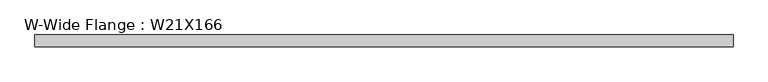
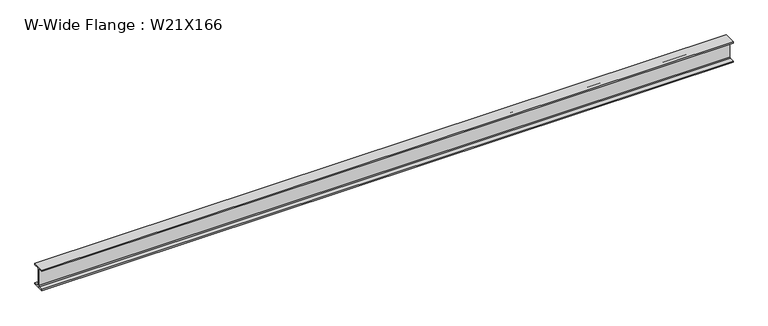
"""IFC4 building model written with IfcOpenShell, lengths in millimetres: beam geometry, W-Wide Flange : W21X166."""

from ifc_helpers import new_model, si_unit, point, frame, frame_2d, origin, place, context, project, spatial, polyline, circle_curve, trimmed, segment, composite_curve, outline, extrude, source, transform, mapped, element, save


def w_wide_flange_w21x166_b0166a6a(model_context):
    return source(origin(), model_context, "Body", "SweptSolid", [
        extrude(outline(composite_curve([segment(polyline([(157.48, -251.206), (157.48, -285.75), (-157.48, -285.75), (-157.48, -251.206), (-32.131, -251.206)]), True, "CONTINUOUS"), segment(trimmed(circle_curve(frame_2d((-32.131, -228.6)), 22.606), [point((-32.131, -251.206))], [point((-9.525, -228.6))], True, "CARTESIAN"), True, "CONTINUOUS"), segment(polyline([(-9.525, -228.6), (-9.525, 228.6)]), True, "CONTINUOUS"), segment(trimmed(circle_curve(frame_2d((-32.131, 228.6)), 22.606), [point((-9.525, 228.6))], [point((-32.131, 251.206))], True, "CARTESIAN"), True, "CONTINUOUS"), segment(polyline([(-32.131, 251.206), (-157.48, 251.206), (-157.48, 285.75), (157.48, 285.75), (157.48, 251.206), (32.131, 251.206)]), True, "CONTINUOUS"), segment(trimmed(circle_curve(frame_2d((32.131, 228.6)), 22.606), [point((32.131, 251.206))], [point((9.525, 228.6))], True, "CARTESIAN"), True, "CONTINUOUS"), segment(polyline([(9.525, 228.6), (9.525, -228.6)]), True, "CONTINUOUS"), segment(trimmed(circle_curve(frame_2d((32.131, -228.6)), 22.606), [point((9.525, -228.6))], [point((32.131, -251.206))], True, "CARTESIAN"), True, "CONTINUOUS"), segment(polyline([(32.131, -251.206), (157.48, -251.206)]), True, "CONTINUOUS")], self_intersect=False)), frame((-9106.3295465, 0.0, 0.0), z_axis=(1.0, 0.0, 0.0), x_axis=(0.0, 1.0, 0.0)), (0.0, 0.0, 1.0), 18197.9516916),
    ])


if __name__ == "__main__":
    model = new_model("IFC4")
    model_context = context("Model", 3, world=origin())
    ifc_project = project(units=[si_unit("LENGTHUNIT", "METRE", prefix="MILLI")], contexts=[model_context])
    site = spatial("IfcSite", under=ifc_project)
    building = spatial("IfcBuilding", under=site)
    placement = place(None, origin())
    w_wide_flange_w21x166_shape = w_wide_flange_w21x166_b0166a6a(model_context)
    element("IfcBeam", 1, ObjectType="W-Wide Flange : W21X166", at=placement, inside=building, context=model_context, shape_type="MappedRepresentation", body=[
        mapped(w_wide_flange_w21x166_shape, transform((0.0, 0.0, 0.0), x_axis=(1.0, 0.0, 0.0), y_axis=(0.0, 1.0, 0.0), z_axis=(0.0, 0.0, 1.0))),
    ])
    save(model, "model.ifc")

# Revit data of these elements
# Type "W-Wide Flange : W21X166"
#   Assembly Code = "B10"
#   W = 166
#   Length [instance default] = 5' - 0"
#   bf = 1' - 0.4"
#   d = 1' - 10 1/2"
#   k = 0' - 2 1/4"
#   k2 = 0' - 0.89"
#   tf = 0' - 1.36"
#   tw = 0' - 0 3/4"
#   A = 0.338889 SF
#   Structural Material [instance default] = Steel ASTM A992
# Element 1 (IfcBeam, "W-Wide Flange : W21X166")
#   Structural Material = Steel
#   Materials on its faces: "Steel"
# Materials
#   "Steel ASTM A992": class "Metal", colour RGB 199 199 199, transparency 0, Description = "Structural steel 50ksi", Cost = 0
#   "Steel": class "Metal", colour RGB 118 118 114, transparency 0, Description = "Steel, mill finish", Cost = 0
